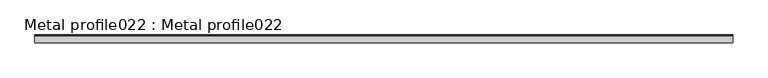
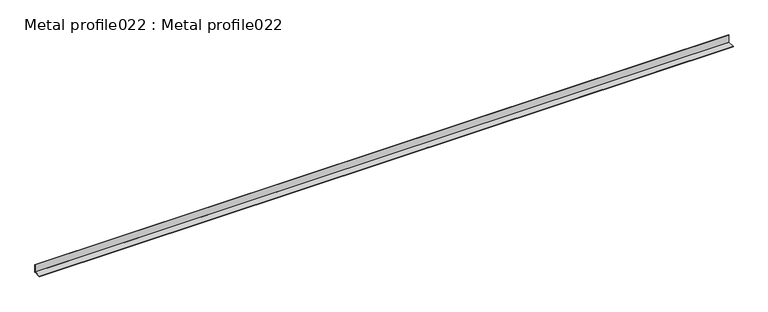
"""IFC4 building model written with IfcOpenShell, lengths in millimetres: proxy geometry, Metal profile022 : Metal profile022."""

from ifc_helpers import new_model, si_unit, point, frame, frame_2d, origin, place, context, project, spatial, polyline, circle_curve, trimmed, segment, composite_curve, outline, extrude, source, transform, mapped, element, save


def metal_profile022_metal_profile022_fb241e4e(model_context):
    return source(origin(), model_context, "Body", "SweptSolid", [
        extrude(outline(composite_curve([segment(polyline([(-4483.2475368, 39025.6541813), (-4481.9675368, 39025.6541813), (-4481.9675368, 39004.7512716)]), True, "CONTINUOUS"), segment(trimmed(circle_curve(frame_2d((-4482.6075368, 39003.8609974)), 1.0964434), [point((-4481.9675368, 39004.7512716))], [point((-4483.497811, 39003.2209974))], False, "CARTESIAN"), True, "CONTINUOUS"), segment(polyline([(-4483.497811, 39003.2209974), (-4504.4007207, 39003.2209974), (-4504.4007207, 39004.5009974), (-4483.2475368, 39004.5009974), (-4483.2475368, 39025.6541813)]), True, "CONTINUOUS")], self_intersect=False)), frame((12383.0178845, 0.0, 0.0), z_axis=(1.0, 0.0, 0.0), x_axis=(0.0, 1.0, 0.0)), (0.0, 0.0, 1.0), 2000.0),
    ])


if __name__ == "__main__":
    model = new_model("IFC4")
    model_context = context("Model", 3, world=origin())
    ifc_project = project(units=[si_unit("LENGTHUNIT", "METRE", prefix="MILLI")], contexts=[model_context])
    site = spatial("IfcSite", under=ifc_project)
    building = spatial("IfcBuilding", under=site)
    placement = place(None, origin())
    metal_profile022_metal_profile022_shape = metal_profile022_metal_profile022_fb241e4e(model_context)
    element("IfcBuildingElementProxy", 1, Name="Metal profile022 : Metal profile022", ObjectType="Metal profile022 : Metal profile022", at=placement, inside=building, context=model_context, shape_type="MappedRepresentation", body=[
        mapped(metal_profile022_metal_profile022_shape, transform((0.0, 0.0, 0.0), x_axis=(1.0, 0.0, 0.0), y_axis=(0.0, 1.0, 0.0), z_axis=(0.0, 0.0, 1.0))),
    ])
    save(model, "model.ifc")

# Revit data of these elements
# Type "Metal profile022 : Metal profile022"
#   NameOverride = "Metal profile022"
# Element 1 (IfcBuildingElementProxy, "Metal profile022 : Metal profile022")
#   Materials on its faces: "CORNER BEAD"
# Materials
#   "CORNER BEAD": class "Unassigned", colour RGB 255 241 0, transparency 0
